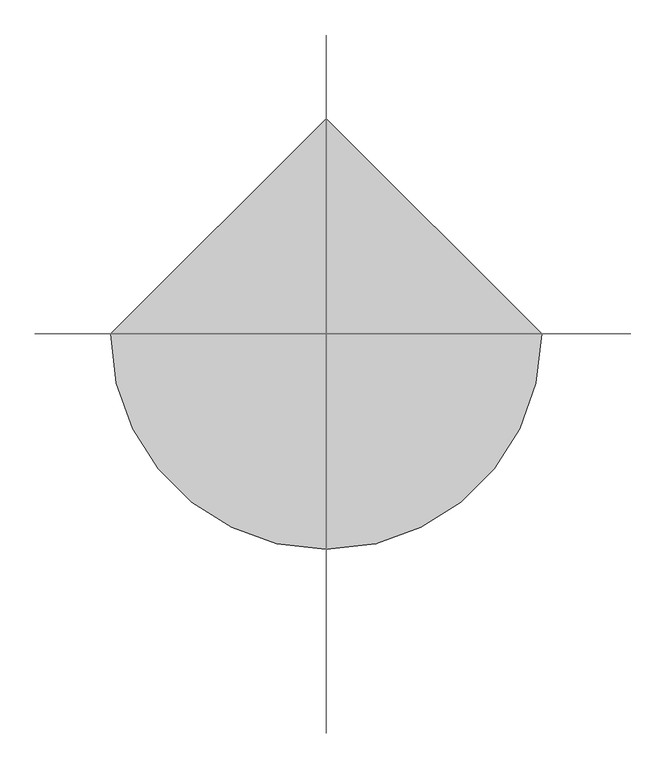
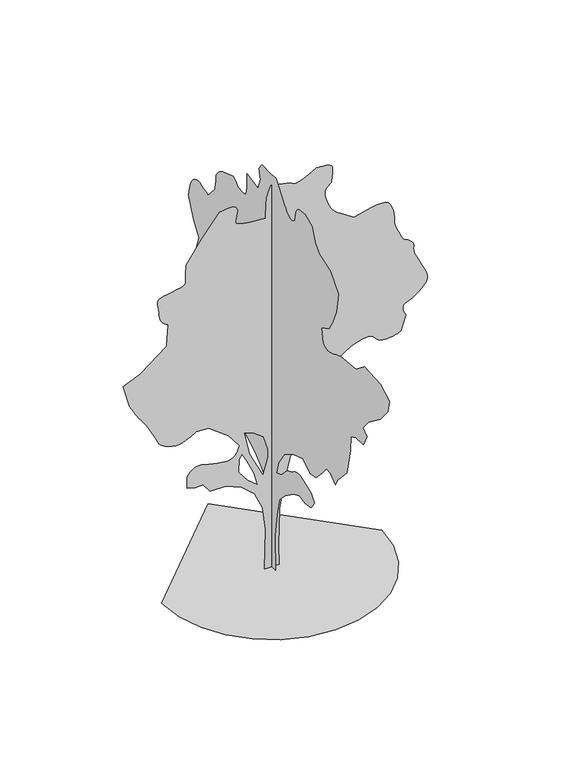
"""IFC4 building model written with IfcOpenShell, lengths in millimetres: proxy geometry, japanese flowering cherry 26172 : japanese flowering cherry 26172."""

import ifcopenshell
import ifcopenshell.guid

model = None  # the IFC model being written
_history = None  # IfcOwnerHistory: only IFC2X3 demands one
_inside = {}  # id of a spatial element -> (the spatial element, [elements in it])
_under = {}  # id of a project, library or spatial element -> (it, [spatial elements below it])
_declared = {}  # id of a project -> (the project, [libraries it declares])
_typed = {}  # id of a type object -> (the type object, [elements of that type])
_made_of = {}  # id of a material, layer set ... -> (it, [elements and type objects made of it])


def new_model(schema):
    """Start an empty IFC model of exactly this schema.

    Asked for "IFC4X3", IfcOpenShell would pick the latest addendum, in which some entities
    have other attributes; the version numbers below select the first issue.
    IFC2X3 requires an IfcOwnerHistory on every rooted entity: one is made here for all.
    """
    global model, _history
    if schema == "IFC4X3":
        model = ifcopenshell.file(schema_version=(4, 3, 0, 0))
    else:
        model = ifcopenshell.file(schema=schema)
    _inside.clear()
    _under.clear()
    _declared.clear()
    _typed.clear()
    _made_of.clear()
    _history = None
    if model.schema == "IFC2X3":
        org = make("IfcOrganization", Name="unknown")
        user = make(
            "IfcPersonAndOrganization",
            ThePerson=make("IfcPerson", FamilyName="unknown"),
            TheOrganization=org,
        )
        app = make(
            "IfcApplication",
            ApplicationDeveloper=org,
            Version="unknown",
            ApplicationFullName="unknown",
            ApplicationIdentifier="unknown",
        )
        _history = make(
            "IfcOwnerHistory",
            OwningUser=user,
            OwningApplication=app,
            ChangeAction="ADDED",
            CreationDate=0,
        )
    return model


def make(cls, **values):
    """One entity of the class cls with the attributes given. An attribute that is None is left unset."""
    return model.create_entity(
        cls, **{name: value for name, value in values.items() if value is not None}
    )


def rooted(cls, **values):
    """An entity with a GlobalId (a new one), such as an element, a storey or a relation."""
    return make(cls, GlobalId=ifcopenshell.guid.new(), OwnerHistory=_history, **values)


def si_unit(unit_type, name, prefix=None):
    """IfcSIUnit, for example si_unit("LENGTHUNIT", "METRE", prefix="MILLI")."""
    return make("IfcSIUnit", UnitType=unit_type, Prefix=prefix, Name=name)


def assignment(units):
    """IfcUnitAssignment: the units of a project."""
    return None if units is None else make("IfcUnitAssignment", Units=units)


def point(xyz):
    """IfcCartesianPoint."""
    return None if xyz is None else make("IfcCartesianPoint", Coordinates=xyz)


def direction(xyz):
    """IfcDirection."""
    return None if xyz is None else make("IfcDirection", DirectionRatios=xyz)


def frame(location, z_axis=None, x_axis=None):
    """IfcAxis2Placement3D, a coordinate frame: its origin and axes. An axis left out is left unset."""
    return make(
        "IfcAxis2Placement3D",
        Location=point(location),
        Axis=direction(z_axis),
        RefDirection=direction(x_axis),
    )


def origin():
    """The frame at (0, 0, 0) with its axes left unset."""
    return frame((0.0, 0.0, 0.0))


def place(relative_to, where):
    """IfcLocalPlacement: puts the frame where relative to a parent placement (None: the world)."""
    return make(
        "IfcLocalPlacement", PlacementRelTo=relative_to, RelativePlacement=where
    )


def context(
    kind, dimensions, precision=None, world=None, true_north=None, identifier=None
):
    """IfcGeometricRepresentationContext, for example the 3D "Model" context."""
    return make(
        "IfcGeometricRepresentationContext",
        ContextIdentifier=identifier,
        ContextType=kind,
        CoordinateSpaceDimension=dimensions,
        Precision=precision,
        WorldCoordinateSystem=world,
        TrueNorth=true_north,
    )


def project(units=None, contexts=None):
    """IfcProject with its units and contexts."""
    return rooted(
        "IfcProject",
        Name="project",
        RepresentationContexts=contexts,
        UnitsInContext=assignment(units),
    )


def spatial(cls, under=None, at=None, **own):
    """A site, building, storey or space (cls), placed at a placement, below another one or the project."""
    s = rooted(cls, ObjectPlacement=at, **own)
    if under is not None:
        _under.setdefault(under.id(), (under, []))[1].append(s)
    return s


def point_list(points):
    """IfcCartesianPointList2D or 3D."""
    cls = (
        "IfcCartesianPointList2D" if len(points[0]) == 2 else "IfcCartesianPointList3D"
    )
    return make(cls, CoordList=points)


def triangles(points, corners, closed=None, point_numbers=None):
    """IfcTriangulatedFaceSet: each triangle names its three corners, points numbered from 1."""
    return make(
        "IfcTriangulatedFaceSet",
        Coordinates=point_list(points),
        Closed=closed,
        CoordIndex=corners,
        PnIndex=point_numbers,
    )


def shape(context_of_items, identifier, shape_type, items):
    """IfcShapeRepresentation: the items that make up one representation, for example the "Body"."""
    return make(
        "IfcShapeRepresentation",
        ContextOfItems=context_of_items,
        RepresentationIdentifier=identifier,
        RepresentationType=shape_type,
        Items=items,
    )


def source(mapping_origin, context_of_items, identifier, shape_type, items):
    """IfcRepresentationMap: a shape defined once, which mapped items show again and again."""
    return make(
        "IfcRepresentationMap",
        MappingOrigin=mapping_origin,
        MappedRepresentation=shape(context_of_items, identifier, shape_type, items),
    )


def transform(
    local_origin,
    x_axis=None,
    y_axis=None,
    z_axis=None,
    scale=None,
    scale2=None,
    scale3=None,
    uniform=True,
):
    """IfcCartesianTransformationOperator3D, or its non-uniform kind. x_axis, y_axis, z_axis: its Axis1, 2, 3."""
    if uniform:
        return make(
            "IfcCartesianTransformationOperator3D",
            Axis1=direction(x_axis),
            Axis2=direction(y_axis),
            LocalOrigin=point(local_origin),
            Scale=scale,
            Axis3=direction(z_axis),
        )
    return make(
        "IfcCartesianTransformationOperator3DnonUniform",
        Axis1=direction(x_axis),
        Axis2=direction(y_axis),
        LocalOrigin=point(local_origin),
        Scale=scale,
        Axis3=direction(z_axis),
        Scale2=scale2,
        Scale3=scale3,
    )


def mapped(mapping_source, mapping_target):
    """IfcMappedItem: shows the shape of a source again, moved by a transform."""
    return make(
        "IfcMappedItem", MappingSource=mapping_source, MappingTarget=mapping_target
    )


def made_of(thing, what):
    """Note that an element or type object is made of a material, layer set ...; save() writes the relation."""
    if what is not None:
        _made_of.setdefault(what.id(), (what, []))[1].append(thing)
    return thing


def element(
    cls,
    number,
    at=None,
    inside=None,
    cuts=None,
    type_object=None,
    material=None,
    context=None,
    identifier="Body",
    shape_type=None,
    held_by="IfcProductDefinitionShape",
    body=None,
    shapes=None,
    **own,
):
    """One element of the class cls, such as IfcWall. Its Tag is "e" and its number.

    at: its placement. inside: the storey or other place that contains it. cuts: it is an
    opening in that element (IfcRelVoidsElement). A single representation is given by context,
    identifier, shape_type and body (its items); several are given by shapes. held_by: the class
    of the entity that holds the representations. save() writes the other relations.
    """
    e = rooted(cls, Tag="e%d" % number, ObjectPlacement=at, **own)
    if body is not None:
        shapes = [shape(context, identifier, shape_type, body)]
    if shapes is not None:
        e.Representation = make(held_by, Representations=shapes)
    if inside is not None:
        _inside.setdefault(inside.id(), (inside, []))[1].append(e)
    if cuts is not None:
        rooted(
            "IfcRelVoidsElement", RelatingBuildingElement=cuts, RelatedOpeningElement=e
        )
    if type_object is not None:
        _typed.setdefault(type_object.id(), (type_object, []))[1].append(e)
    return made_of(e, material)


def aggregate(whole, parts):
    """IfcRelAggregates: a whole, such as a stair, and the parts it consists of."""
    return rooted("IfcRelAggregates", RelatingObject=whole, RelatedObjects=parts)


def save(model, path):
    """Write the relations noted so far, then the file.

    IfcRelAggregates (storeys below a building ...), IfcRelContainedInSpatialStructure (elements
    in a storey), IfcRelDefinesByType, IfcRelAssociatesMaterial and IfcRelDeclares: one each for
    every whole, place, type object, material and project.
    """
    for whole, parts in _under.values():
        aggregate(whole, parts)
    for where, things in _inside.values():
        rooted(
            "IfcRelContainedInSpatialStructure",
            RelatedElements=things,
            RelatingStructure=where,
        )
    for kind, things in _typed.values():
        rooted("IfcRelDefinesByType", RelatedObjects=things, RelatingType=kind)
    for what, things in _made_of.values():
        rooted("IfcRelAssociatesMaterial", RelatedObjects=things, RelatingMaterial=what)
    for by, libraries in _declared.values():
        rooted("IfcRelDeclares", RelatingContext=by, RelatedDefinitions=libraries)
    model.write(path)


def entourage_e499737d(model_context):
    return source(origin(), model_context, "Body", "Tessellation", [
        triangles([(-0.0028028, 75.7657196, 0.0059537), (-0.0028028, -73.2478183, 0.0059537), (-0.0028028, -59.7012251, 399.6312029), (-0.0028028, -100.3410047, 663.7914597), (-0.0028028, -147.7544623, 866.9916292), (-0.0028028, -256.1287339, 982.1375078), (-0.0028028, -418.6863261, 1097.2859299), (-0.0028028, -527.0605977, 1144.6976435), (-0.0028028, -635.434833, 1124.3775902), (-0.0028028, -750.5807842, 1144.6976435), (-0.0028028, -811.5407988, 1232.7519344), (-0.0028028, -750.5807842, 1314.0320023), (-0.0028028, -533.8347845, 1388.5377743), (-0.0028028, -514.9955638, 1387.0189716), (-0.0028028, -496.3341665, 1385.0834793), (-0.0028028, -478.0283798, 1382.3173691), (-0.0028028, -460.2559908, 1378.3091835), (-0.0028028, -443.1947865, 1372.6425236), (-0.0028028, -427.0200471, 1364.9005543), (-0.0028028, -411.9146828, 1354.6719635), (-0.0028028, -396.8067387, 1343.65345), (-0.0028028, -380.6345427, 1333.6991158), (-0.0028028, -363.5733384, 1324.6364422), (-0.0028028, -345.8009494, 1316.2824463), (-0.0028028, -327.4951627, 1308.4643188), (-0.0028028, -308.8337654, 1300.9992222), (-0.0028028, -289.994581, 1293.7118763), (-0.0028028, -188.3942419, 1185.3376774), (-0.0028028, -86.7944115, 1144.6976435), (-0.0028028, -127.4344454, 1286.9377258), (-0.0028028, -242.580869, 1456.2720119), (-0.0028028, -405.140496, 1557.8722057), (-0.0028028, -594.794799, 1618.8321476), (-0.0028028, -730.2607309, 1530.7779293), (-0.0028028, -838.6350025, 1544.3263756), (-0.0028028, -953.7809538, 1666.2439339), (-0.0028028, -1041.8351721, 1774.6181328), (-0.0028028, -1123.1126965, 1767.8439823), (-0.0028028, -1211.1669147, 1686.5663853), (-0.0028028, -1265.3528515, 1781.3922832), (-0.0028028, -1326.3127934, 1849.1240501), (-0.0028028, -1434.6871376, 1964.2723995), (-0.0028028, -1502.4187592, 2269.0726902), (-0.0028028, -1509.193055, 2431.6328259), (-0.0028028, -1604.0214237, 2472.2703163), (-0.0028028, -1753.0332584, 2485.8186172), (-0.0028028, -1813.9932003, 2614.5002975), (-0.0028028, -1739.4874283, 2675.4602394), (-0.0028028, -1841.0874767, 2797.3804138), (-0.0028028, -2071.3792339, 2973.5042564), (-0.0028028, -2220.3935394, 3149.6025192), (-0.0028028, -2247.4851997, 3291.8426743), (-0.0028028, -2078.1535297, 3386.6610146), (-0.0028028, -1766.5790886, 3400.2244308), (-0.0028028, -1610.7931034, 3278.3045471), (-0.0028028, -1312.7669632, 3244.4208595), (-0.0028028, -1272.2845505, 3228.5456657), (-0.0028028, -1232.7519344, 3213.2041603), (-0.0028028, -1195.1115721, 3198.9294502), (-0.0028028, -1160.3186377, 3186.2546425), (-0.0028028, -1129.3153702, 3175.7137161), (-0.0028028, -1103.0517843, 3167.8397781), (-0.0028028, -1082.4726625, 3163.1406464), (-0.0028028, -1064.0500225, 3162.8865921), (-0.0028028, -1044.5580437, 3166.9000099), (-0.0028028, -1025.4242552, 3173.6309944), (-0.0028028, -1008.065867, 3181.5558014), (-0.0028028, -993.907865, 3189.1248161), (-0.0028028, -984.3701477, 3194.789296), (-0.0028028, -980.8726141, 3197.024334), (-0.0028028, -947.0067307, 3359.5844696), (-0.0028028, -1089.2468857, 3434.0828293), (-0.0028028, -1156.9810507, 3542.4645859), (-0.0028028, -1231.4868954, 3718.5628487), (-0.0028028, -1272.127002, 3942.0832169), (-0.0028028, -1116.3410168, 4118.1814796), (-0.0028028, -913.1409199, 4192.7051285), (-0.0028028, -831.8608521, 4267.2034882), (-0.0028028, -770.9007648, 4429.7636238), (-0.0028028, -628.6606825, 4483.9417122), (-0.0028028, -605.4958537, 4483.8402649), (-0.0028028, -582.6891789, 4483.1542603), (-0.0028028, -560.5911455, 4481.2747238), (-0.0028028, -539.5599438, 4477.6426781), (-0.0028028, -519.9511116, 4471.5974075), (-0.0028028, -502.1202959, 4462.6310944), (-0.0028028, -486.4205638, 4450.0836044), (-0.0028028, -473.6824242, 4434.3863068), (-0.0028028, -464.1447433, 4416.5554184), (-0.0028028, -457.2740144, 4396.9467316), (-0.0028028, -452.5343691, 4375.9154572), (-0.0028028, -449.3949532, 4353.8173874), (-0.0028028, -447.3197528, 4331.0083145), (-0.0028028, -445.7805299, 4307.8434494), (-0.0028028, -434.0914178, 4294.9401672), (-0.0028028, -421.9248276, 4283.0531021), (-0.0028028, -408.8133096, 4273.1978897), (-0.0028028, -394.279422, 4266.3398781), (-0.0028028, -377.850701, 4263.5202827), (-0.0028028, -359.0495956, 4265.7303223), (-0.0028028, -337.4062583, 4273.9853416), (-0.0028028, -315.9610193, 4285.9741447), (-0.0028028, -297.7161846, 4298.6995308), (-0.0028028, -282.1358129, 4312.0091835), (-0.0028028, -268.6864885, 4325.8013649), (-0.0028028, -256.8373934, 4339.9237587), (-0.0028028, -246.0563473, 4354.3002068), (-0.0028028, -235.8074452, 4368.8033913), (-0.0028028, -140.9810386, 4497.5054192), (-0.0028028, -80.0209877, 4572.0037788), (-0.0028028, 21.579147, 4565.2219254), (-0.0028028, 184.1389784, 4572.0037788), (-0.0028028, 245.0987749, 4490.7235657), (-0.0028028, 218.0055885, 4375.5852448), (-0.0028028, 265.4200454, 4246.8835075), (-0.0028028, 475.3918765, 4287.5234688), (-0.0028028, 475.3918765, 4138.5014603), (-0.0028028, 476.9514107, 4115.4383331), (-0.0028028, 479.1637756, 4093.1623672), (-0.0028028, 482.6791134, 4072.5630432), (-0.0028028, 488.1502911, 4054.4781006), (-0.0028028, 496.2249435, 4039.6699928), (-0.0028028, 507.5609885, 4029.0273285), (-0.0028028, 522.8060609, 4023.3631393), (-0.0028028, 540.2228757, 4021.2551285), (-0.0028028, 557.6396542, 4020.5691238), (-0.0028028, 575.056469, 4021.0519432), (-0.0028028, 592.4732474, 4022.4995293), (-0.0028028, 609.8900259, 4024.6586998), (-0.0028028, 627.3093842, 4027.2748192), (-0.0028028, 644.726199, 4030.1449928), (-0.0028028, 660.7002239, 4045.9437378), (-0.0028028, 676.7352917, 4060.8791634), (-0.0028028, 692.8896835, 4074.0362091), (-0.0028028, 709.2193554, 4084.5265572), (-0.0028028, 725.7878208, 4091.4607269), (-0.0028028, 742.6534338, 4093.9498192), (-0.0028028, 759.8720776, 4091.1049347), (-0.0028028, 942.7522665, 4030.1449928), (-0.0028028, 968.7009007, 4012.6698967), (-0.0028028, 993.5827394, 3994.8390083), (-0.0028028, 1016.3309875, 3976.2971169), (-0.0028028, 1035.8813931, 3956.6881393), (-0.0028028, 1051.1646172, 3935.6568649), (-0.0028028, 1061.1163353, 3912.8477921), (-0.0028028, 1064.6722956, 3887.9048378), (-0.0028028, 1065.462291, 3862.3526184), (-0.0028028, 1067.6745832, 3837.8921928), (-0.0028028, 1071.0705969, 3814.3209572), (-0.0028028, 1075.4140091, 3791.4610153), (-0.0028028, 1080.4685698, 3769.1088913), (-0.0028028, 1085.9981741, 3747.1381393), (-0.0028028, 1091.7640285, 3725.3447021), (-0.0028028, 1220.4582081, 3583.1045471), (-0.0028028, 1259.5970982, 3600.2497215), (-0.0028028, 1298.4413841, 3615.8705704), (-0.0028028, 1336.691375, 3628.418351), (-0.0028028, 1374.0521759, 3636.343158), (-0.0028028, 1410.2294735, 3638.0956673), (-0.0028028, 1444.9259022, 3632.1521347), (-0.0028028, 1477.8442417, 3616.9629456), (-0.0028028, 1506.4193871, 3593.4931572), (-0.0028028, 1528.9517326, 3564.3086014), (-0.0028028, 1546.4471764, 3530.3996246), (-0.0028028, 1559.9143776, 3492.7059952), (-0.0028028, 1570.361269, 3452.1674812), (-0.0028028, 1578.7941845, 3409.7241417), (-0.0028028, 1586.218586, 3366.3410339), (-0.0028028, 1498.1643677, 3136.0643921), (-0.0028028, 1389.7926395, 2987.0423836), (-0.0028028, 1477.8442417, 2743.2023254), (-0.0028028, 1396.5641739, 2614.5002975), (-0.0028028, 1363.3893093, 2602.8164177), (-0.0028028, 1331.4588455, 2590.6497185), (-0.0028028, 1302.0151485, 2577.543251), (-0.0028028, 1276.3027645, 2563.0144867), (-0.0028028, 1255.5687103, 2546.5806061), (-0.0028028, 1241.0552067, 2527.7820442), (-0.0028028, 1234.0040382, 2506.1385979), (-0.0028028, 1231.6953129, 2483.1135498), (-0.0028028, 1230.4506214, 2460.4416779), (-0.0028028, 1230.0949745, 2438.0692062), (-0.0028028, 1230.4506214, 2415.9330574), (-0.0028028, 1231.339666, 2393.9721886), (-0.0028028, 1232.5842121, 2372.13326), (-0.0028028, 1234.0040382, 2350.3502872), (-0.0028028, 1206.9124506, 2241.9785591), (-0.0028028, 1017.2581112, 2262.2985397), (-0.0028028, 1001.4999161, 2230.5052769), (-0.0028028, 986.9863398, 2199.5401611), (-0.0028028, 974.9594576, 2170.2361359), (-0.0028028, 966.6663591, 2143.4188774), (-0.0028028, 963.3491198, 2119.9211838), (-0.0028028, 966.2523582, 2100.5664059), (-0.0028028, 976.6180773, 2086.1925739), (-0.0028028, 993.4227201, 2074.2646683), (-0.0028028, 1014.0196461, 2062.1005852), (-0.0028028, 1037.2225176, 2050.292149), (-0.0028028, 1061.8478313, 2039.431184), (-0.0028028, 1086.7093952, 2030.1093693), (-0.0028028, 1110.6234879, 2022.9211452), (-0.0028028, 1132.4039898, 2018.4583363), (-0.0028028, 1152.1322187, 2014.567004), (-0.0028028, 1170.7936523, 2008.9003441), (-0.0028028, 1188.5660414, 2001.7526699), (-0.0028028, 1205.6272093, 1993.4190216), (-0.0028028, 1222.157523, 1984.1961834), (-0.0028028, 1238.3297916, 1974.3816662), (-0.0028028, 1254.3241642, 1964.2723995), (-0.0028028, 1410.1126202, 2045.5524673), (-0.0028028, 1454.8979679, 2056.9850544), (-0.0028028, 1498.4412403, 2067.3533169), (-0.0028028, 1539.4952751, 2075.5879887), (-0.0028028, 1576.817997, 2080.6222744), (-0.0028028, 1609.1650051, 2081.3919949), (-0.0028028, 1635.2914627, 2076.8326801), (-0.0028028, 1653.9502075, 2065.8725933), (-0.0028028, 1666.2946575, 2049.9747265), (-0.0028028, 1674.7249569, 2031.5900928), (-0.0028028, 1679.8989143, 2011.1329113), (-0.0028028, 1682.4669262, 1989.0146393), (-0.0028028, 1683.0789528, 1965.6542919), (-0.0028028, 1682.3881519, 1941.4631813), (-0.0028028, 1681.0444839, 1916.8582878), (-0.0028028, 1657.7627655, 1892.3904499), (-0.0028028, 1634.1255455, 1869.1697742), (-0.0028028, 1609.7770317, 1848.4331039), (-0.0028028, 1584.3618679, 1831.4303627), (-0.0028028, 1557.5241165, 1819.4059513), (-0.0028028, 1528.9110374, 1813.5996197), (-0.0028028, 1498.1643677, 1815.2582394), (-0.0028028, 1465.6015297, 1822.4057682), (-0.0028028, 1432.5637207, 1830.9782101), (-0.0028028, 1400.2370602, 1839.0732101), (-0.0028028, 1369.8078129, 1844.8009129), (-0.0028028, 1342.4571568, 1846.2614342), (-0.0028028, 1319.3735367, 1841.5624477), (-0.0028028, 1301.7382759, 1828.8040695), (-0.0028028, 1288.4084209, 1812.3752758), (-0.0028028, 1277.2120113, 1797.7219551), (-0.0028028, 1267.7912201, 1784.5521194), (-0.0028028, 1259.7953419, 1772.5657871), (-0.0028028, 1252.8636429, 1761.4660286), (-0.0028028, 1246.6430923, 1750.9605652), (-0.0028028, 1240.778334, 1740.752322), (-0.0028028, 1263.8618088, 1737.6916077), (-0.0028028, 1286.1172817, 1733.6834221), (-0.0028028, 1306.714135, 1727.7779686), (-0.0028028, 1324.821896, 1719.0302467), (-0.0028028, 1339.6122723, 1706.4901691), (-0.0028028, 1350.2574074, 1689.2105553), (-0.0028028, 1355.9242126, 1666.2439339), (-0.0028028, 1358.2355541, 1639.3300243), (-0.0028028, 1359.4802456, 1610.9912018), (-0.0028028, 1359.8357471, 1581.4687305), (-0.0028028, 1359.4802456, 1550.9989334), (-0.0028028, 1358.591201, 1519.8178425), (-0.0028028, 1357.3466549, 1488.1643967), (-0.0028028, 1355.9242126, 1456.2720119), (-0.0028028, 1321.1312782, 1430.3436527), (-0.0028028, 1286.5720505, 1405.5990875), (-0.0028028, 1252.4876484, 1383.2266159), (-0.0028028, 1219.1146128, 1364.4078518), (-0.0028028, 1186.6915192, 1350.328624), (-0.0028028, 1155.4494581, 1342.1725811), (-0.0028028, 1125.6323828, 1341.1261333), (-0.0028028, 1095.812764, 1344.8167511), (-0.0028028, 1064.5732464, 1349.9322819), (-0.0028028, 1032.1476093, 1356.2316067), (-0.0028028, 998.774501, 1363.478112), (-0.0028028, 964.6902443, 1371.4385273), (-0.0028028, 930.1334873, 1379.8688267), (-0.0028028, 895.3380095, 1388.5377743), (-0.0028028, 692.1378399, 1341.1261333), (-0.0028028, 455.0718596, 1219.2061043), (-0.0028028, 319.6059277, 1144.6976435), (-0.0028028, 163.8189614, 1016.005862), (-0.0028028, 68.9922959, 819.5799156), (-0.0028028, 41.8991095, 541.8713216), (-0.0028028, 68.9922959, 264.1652892), (80.2102203, 0.0002552, 0.0), (-82.349661, 0.0002552, 0.0), (-68.8030678, 0.0002233, 460.5862032), (-102.6694236, 0.000202, 724.7463873), (-190.7229152, 0.0001914, 914.3981833), (-332.9637969, 0.0001914, 1043.0925081), (-509.0697627, 0.0001807, 1117.5983528), (-678.4015417, 0.0001807, 1117.5983528), (-759.684153, 0.0001807, 1219.1984013), (-847.7358278, 0.0001807, 1219.1984013), (-935.7901188, 0.0001807, 1239.5183819), (-935.7901188, 0.0001701, 1368.2127068), (-918.2539072, 0.0001701, 1391.2175526), (-900.0065472, 0.0001701, 1412.9192802), (-880.3392883, 0.0001595, 1432.0150623), (-858.5384388, 0.0001595, 1447.2017807), (-833.8928501, 0.0001595, 1457.1737011), (-805.6936993, 0.0001595, 1460.6307575), (-773.2299831, 0.0001595, 1456.266925), (-734.6829174, 0.0001595, 1446.5108345), (-690.4487715, 0.0001595, 1435.4516258), (-643.1335636, 0.0001701, 1424.2757092), (-595.3460009, 0.0001701, 1414.1639717), (-549.689449, 0.0001701, 1406.3051491), (-508.7725788, 0.0001701, 1401.8804192), (-475.2013721, 0.0001701, 1402.0785175), (-448.544024, 0.0001701, 1408.1415195), (-426.1513865, 0.0001701, 1419.8916744), (-407.3122021, 0.0001595, 1436.3813656), (-391.3152497, 0.0001595, 1456.660651), (-377.4544679, 0.0001595, 1479.7848209), (-365.0135485, 0.0001595, 1504.8039333), (-353.2838139, 0.0001595, 1530.7728424), (-475.2013721, 0.0001488, 1693.3329781), (-698.7215223, 0.0001382, 1855.8931137), (-834.1899977, 0.0001382, 1862.6647934), (-856.0492739, 0.0001382, 1849.6320133), (-878.4419477, 0.0001382, 1836.7771294), (-901.9038877, 0.0001382, 1824.277747), (-926.9610065, 0.0001382, 1812.3092915), (-954.1543322, 0.0001382, 1801.0544552), (-984.01203, 0.0001382, 1790.6861927), (-1017.0701866, 0.0001488, 1781.3847256), (-1055.1015862, 0.0001488, 1778.1664627), (-1097.4002398, 0.0001488, 1784.6638859), (-1140.7656887, 0.0001382, 1798.9792912), (-1182.0000904, 0.0001382, 1819.2206429), (-1217.9005154, 0.0001382, 1843.490237), (-1245.2690483, 0.0001382, 1869.8935673), (-1260.907774, 0.0001382, 1896.5332203), (-1274.5551968, 0.0001382, 1929.7461639), (-1296.2570698, 0.0001276, 1973.9803825), (-1323.2903034, 0.0001276, 2024.4959038), (-1352.9320988, 0.0001276, 2076.5482498), (-1382.45457, 0.0001276, 2125.4025352), (-1409.1321568, 0.0001169, 2166.3195145), (-1430.2420601, 0.0001169, 2194.5592152), (-1448.055217, 0.0001169, 2217.0508656), (-1466.5769062, 0.0001169, 2243.4541958), (-1485.6928905, 0.0001169, 2273.113868), (-1505.2813751, 0.0001169, 2305.3794857), (-1525.2255066, 0.0001063, 2339.6035595), (-1545.4082863, 0.0001063, 2375.12799), (-1565.7080647, 0.0001063, 2411.3051422), (-1640.2164528, 9.57e-05, 2668.7039658), (-1443.7878902, 8.51e-05, 2749.9838882), (-1159.310269, 7.44e-05, 2973.5042564), (-1145.7618954, 5.32e-05, 3217.3190254), (-1165.9447477, 5.32e-05, 3231.9748169), (-1185.2970549, 5.32e-05, 3247.3163223), (-1202.9906696, 5.32e-05, 3264.0804153), (-1218.1951195, 5.32e-05, 3282.9780991), (-1230.0823299, 5.32e-05, 3304.7203766), (-1237.8242992, 5.32e-05, 3330.0188324), (-1240.5902641, 5.32e-05, 3359.5591805), (-1243.0389519, 4.25e-05, 3392.8330215), (-1248.5659401, 4.25e-05, 3427.5294502), (-1254.4511913, 4.25e-05, 3461.7686394), (-1257.9665291, 4.25e-05, 3493.6204742), (-1256.3865383, 4.25e-05, 3521.204837), (-1246.9860947, 4.25e-05, 3542.6169022), (-1227.0419632, 4.25e-05, 3556.002713), (-1192.1092844, 4.25e-05, 3564.4103394), (-1144.1438982, 3.19e-05, 3572.715937), (-1090.0164608, 3.19e-05, 3581.5808029), (-1036.6002445, 3.19e-05, 3591.7915169), (-990.7659056, 3.19e-05, 3603.9835052), (-959.3867163, 3.19e-05, 3618.9186401), (-949.3359489, 3.19e-05, 3637.2829262), (-951.449192, 3.19e-05, 3659.3809959), (-952.1400656, 3.19e-05, 3684.6794518), (-951.644747, 3.19e-05, 3712.6448959), (-950.2045732, 3.19e-05, 3742.718351), (-948.0532511, 2.13e-05, 3774.4175789), (-945.4268852, 2.13e-05, 3807.1836021), (-942.5617258, 2.13e-05, 3840.4830231), (-773.2299831, 1.06e-05, 4084.3233719), (-576.803964, -1.06e-05, 4328.16343), (-534.9980856, -1.06e-05, 4335.1231796), (-494.9117606, -1.06e-05, 4340.3809982), (-458.2595647, -1.06e-05, 4342.2096657), (-426.7635221, -1.06e-05, 4338.8569633), (-402.1382083, -1.06e-05, 4328.6459587), (-386.1031769, -1.06e-05, 4309.850013), (-380.3754742, 0.0, 4280.7416153), (-383.1999384, 0.0, 4247.9503029), (-389.6972889, 0.0, 4219.0450905), (-396.9057878, 0.0, 4193.848082), (-401.8613357, 0.0, 4172.0549355), (-401.6048106, 0.0, 4153.462175), (-393.1720041, 0.0, 4137.8410355), (-373.6038308, 0.0, 4124.9633331), (-343.9238837, 0.0, 4114.5238541), (-307.8431645, 0.0, 4106.2435455), (-266.4335192, 1.06e-05, 4099.7157463), (-220.7586908, 1.06e-05, 4094.6355331), (-171.883967, 1.06e-05, 4090.5971169), (-120.8766607, 1.06e-05, 4087.2697037), (-68.8030678, 1.06e-05, 4084.3233719), (-62.0293897, 0.0, 4267.2034882), (-60.4495079, -1.06e-05, 4293.1367889), (-56.0260951, -1.06e-05, 4318.689299), (-49.2331141, -1.06e-05, 4343.962175), (-40.544273, -1.06e-05, 4369.0065765), (-30.4335416, -1.06e-05, 4393.8733727), (-19.3751868, -1.06e-05, 4418.612851), (-7.8427643, -1.06e-05, 4443.3017509), (38.3857792, -1.06e-05, 4434.5642029), (83.3110485, -1.06e-05, 4425.7249168), (125.6295138, -1.06e-05, 4416.6571564), (164.0381523, -1.06e-05, 4407.2083145), (197.2334371, -1.06e-05, 4397.3022331), (223.9120957, -1.06e-05, 4386.7865959), (242.7705922, -1.06e-05, 4375.5599556), (267.3174405, -1.06e-05, 4372.2834114), (307.2640574, -1.06e-05, 4382.5194145), (355.6256767, -1.06e-05, 4401.5188362), (405.4097383, -1.06e-05, 4424.5566742), (449.6235366, -1.06e-05, 4446.8576385), (481.2770551, -2.13e-05, 4463.7234695), (493.3827115, -2.13e-05, 4470.4035851), (503.1388384, -2.13e-05, 4470.6067703), (528.2975498, -2.13e-05, 4470.3274269), (562.6967946, -2.13e-05, 4468.2699944), (600.177065, -2.13e-05, 4463.1392029), (634.5763098, -1.06e-05, 4453.6142029), (659.7350212, -1.06e-05, 4438.3994339), (669.4911844, -1.06e-05, 4416.1999168), (669.0949877, -1.06e-05, 4390.4698013), (667.9900406, -1.06e-05, 4365.4506889), (666.2907984, -1.06e-05, 4341.0411324), (664.1190559, -1.06e-05, 4317.089106), (661.5918119, -1.06e-05, 4293.4922905), (658.8257017, 0.0, 4270.1245308), (655.9428108, 0.0, 4246.8835075), (638.6835445, 0.0, 4233.6753021), (622.3741476, 0.0, 4219.7308044), (607.9571134, 0.0, 4204.2114029), (596.3848546, 0.0, 4186.4060944), (588.6048426, 0.0, 4165.5271362), (585.5644395, 0.0, 4140.7876579), (588.2111166, 0.0, 4111.3996262), (595.5949319, 1.06e-05, 4078.8367882), (605.8235227, 1.06e-05, 4045.6643944), (618.4244614, 1.06e-05, 4012.9492401), (632.9176901, 1.06e-05, 3981.7834099), (648.8333611, 1.06e-05, 3953.233699), (665.698974, 1.06e-05, 3928.3416138), (683.0370146, 2.13e-05, 3908.1995293), (703.4154945, 2.13e-05, 3889.8099541), (729.1278786, 2.13e-05, 3869.6170006), (759.2802532, 2.13e-05, 3847.9505905), (792.9912043, 2.13e-05, 3825.1159378), (829.3639841, 2.13e-05, 3801.3670967), (867.5148531, 2.13e-05, 3777.0592781), (906.5572374, 2.13e-05, 3752.4212471), (974.48703, 2.13e-05, 3771.0140076), (1040.6997763, 2.13e-05, 3787.8795479), (1103.475959, 2.13e-05, 3801.2909386), (1161.1010027, 2.13e-05, 3809.5712471), (1211.8502306, 2.13e-05, 3810.9682549), (1254.0116833, 2.13e-05, 3803.7800308), (1285.8633728, 2.13e-05, 3786.2793549), (1308.8096466, 2.13e-05, 3757.831382), (1325.9495888, 3.19e-05, 3721.2045479), (1338.1136719, 3.19e-05, 3679.8280037), (1346.1325138, 3.19e-05, 3637.155899), (1350.8315002, 3.19e-05, 3596.6173851), (1353.0438652, 4.25e-05, 3561.641613), (1353.5976105, 4.25e-05, 3535.6827324), (1358.8503422, 4.25e-05, 3507.9969223), (1372.3961723, 4.25e-05, 3469.2870758), (1390.9178616, 4.25e-05, 3425.1418053), (1411.1006413, 5.32e-05, 3381.0982727), (1429.6249466, 5.32e-05, 3342.7442184), (1443.1707767, 5.32e-05, 3315.6423843), (1448.4235085, 5.32e-05, 3305.3808014), (1455.5126106, 5.32e-05, 3302.5614967), (1473.6202263, 5.32e-05, 3294.4079247), (1498.0094353, 5.32e-05, 3281.4031952), (1523.9376492, 5.32e-05, 3264.0042572), (1546.6656223, 5.32e-05, 3242.6936394), (1561.456144, 5.32e-05, 3217.9538704), (1563.5693871, 6.38e-05, 3190.2424805), (1560.9227463, 6.38e-05, 3161.8962456), (1563.9655838, 6.38e-05, 3134.3880409), (1571.7456322, 6.38e-05, 3106.8795456), (1583.3178909, 6.38e-05, 3078.5585999), (1597.7324181, 6.38e-05, 3048.5613029), (1614.0443584, 7.44e-05, 3016.0746231), (1631.3036247, 7.44e-05, 2980.2605301), (1651.0114334, 7.44e-05, 2941.4239471), (1672.8529781, 7.44e-05, 2900.911013), (1693.1526112, 7.44e-05, 2859.5850471), (1708.2377369, 8.51e-05, 2818.2593719), (1714.4404106, 8.51e-05, 2777.7461472), (1708.0801884, 8.51e-05, 2738.9095642), (1685.4894161, 8.51e-05, 2702.5620735), (1655.0603142, 9.57e-05, 2670.8884254), (1626.9983643, 9.57e-05, 2644.9042557), (1600.3587112, 9.57e-05, 2623.6442162), (1574.1941746, 9.57e-05, 2606.1944092), (1547.5546669, 9.57e-05, 2591.5894867), (1519.4951878, 9.57e-05, 2578.8641006), (1489.0634697, 9.57e-05, 2567.103772), (1463.2545799, 9.57e-05, 2553.5147758), (1448.4615875, 9.57e-05, 2536.3646599), (1442.8532089, 9.57e-05, 2516.2632706), (1444.5930737, 0.0001063, 2493.7893517), (1451.8397243, 0.0001063, 2469.5399597), (1462.7592613, 0.0001063, 2444.1069191), (1475.5176395, 0.0001063, 2418.079438), (1421.329232, 0.0001169, 2248.7450066), (1402.2741451, 0.0001169, 2240.1167542), (1382.0913654, 0.0001169, 2231.9607113), (1359.6579964, 0.0001169, 2224.752285), (1333.8491066, 0.0001169, 2218.9661556), (1303.5367126, 0.0001169, 2215.0772942), (1267.5955925, 0.0001169, 2213.5558754), (1224.9032856, 0.0001169, 2214.8791958), (1186.5543182, 0.0001169, 2223.6651421), (1160.2907324, 0.0001169, 2241.2216286), (1139.9504042, 0.0001169, 2263.0426804), (1119.3738258, 0.0001169, 2284.6250839), (1092.3990189, 0.0001169, 2301.470422), (1052.8638594, 0.0001169, 2309.0727196), (994.6089123, 0.0001169, 2302.9309433), (927.2531399, 0.0001169, 2283.7970821), (865.4625074, 0.0001169, 2256.8426228), (810.6645441, 0.0001169, 2224.1985397), (764.2764599, 0.0001169, 2188.0035107), (727.7258566, 0.0001169, 2150.3835686), (702.4274008, 0.0001276, 2113.4772457), (689.8112377, 0.0001276, 2079.4133366), (689.5343651, 0.0001276, 2049.0602474), (699.2092106, 0.0001276, 2021.5520428), (717.179698, 0.0001276, 1996.4136063), (741.7847368, 0.0001276, 1973.172583), (771.3655621, 0.0001382, 1951.3515312), (804.2662428, 0.0001382, 1930.4778053), (838.8229998, 0.0001382, 1910.0790504), (858.9855045, 0.0001382, 1896.9268009), (878.2006107, 0.0001382, 1883.2412991), (895.5183764, 0.0001382, 1868.4914726), (909.9938009, 0.0001382, 1852.1415985), (920.6770878, 0.0001382, 1833.6579884), (926.620693, 0.0001382, 1812.5073898), (926.8772181, 0.0001382, 1788.158876), (924.1721506, 0.0001488, 1758.4790016), (921.8225847, 0.0001488, 1722.4008259), (919.7677683, 0.0001488, 1680.9911442), (917.9516727, 0.0001488, 1635.3142811), (916.3107845, 0.0001595, 1586.4395027), (914.7919092, 0.0001595, 1535.4337498), (913.3288445, 0.0001595, 1483.3585854), (878.4571358, 0.0001595, 1457.529348), (843.3467062, 0.0001595, 1433.4780544), (807.7613056, 0.0001701, 1412.980323), (771.4646839, 0.0001701, 1397.8139523), (734.2231344, 0.0001701, 1389.7570312), (695.792922, 0.0001701, 1390.585033), (655.9428108, 0.0001701, 1402.0785175), (615.8971447, 0.0001701, 1417.3236626), (576.9157305, 0.0001701, 1428.6597439), (538.820781, 0.0001595, 1436.7368671), (501.4395962, 0.0001595, 1442.205574), (464.5917727, 0.0001595, 1445.7209118), (428.0995597, 0.0001595, 1447.9332767), (391.7826267, 0.0001595, 1449.4927746), (276.6366936, 0.0001701, 1374.9868572), (202.1305764, 0.0001807, 1205.6525711), (127.6236689, 0.0001914, 921.1724064), (86.9838894, 0.0002126, 643.4663195), (73.4370464, 0.0002339, 237.0665254), (-95.8962542, 8.51e-05, 1097.2783722), (-41.7096271, 7.44e-05, 1286.9326389), (-41.7096271, 6.38e-05, 1381.7585369), (-89.122576, 5.32e-05, 1544.3186726), (-211.0424234, 5.32e-05, 1632.3728909), (-305.8695931, 5.32e-05, 1666.238847), (-244.9095423, 6.38e-05, 1395.3069832), (-156.8557963, 6.38e-05, 1009.2266247), (-197.4958302, 6.38e-05, 1158.2383867), (-272.003746, 5.32e-05, 1320.7984497), (-326.1896101, 4.25e-05, 1422.3986435), (-360.0554572, 4.25e-05, 1374.9868572), (-366.829644, 5.32e-05, 1225.9725517), (-265.2295592, 6.38e-05, 1097.2783722), (-1212.9170259, 0.0, 0.0045929), (-1180.85205, -277.9194097, 0.0045929), (-1089.5287725, -533.1464181, 0.0045929), (-946.2625174, -758.3633034, 0.0045929), (-758.3633034, -946.2625174, 0.0045929), (-533.1464181, -1089.5287725, 0.0045929), (-277.9194097, -1180.85205, 0.0045929), (5.3e-05, -1212.9170259, 0.0045929), (277.9194097, -1180.85205, 0.0045929), (533.1464181, -1089.5287725, 0.0045929), (758.3633034, -946.2625174, 0.0045929), (946.2625174, -758.3633034, 0.0045929), (1089.5287725, -533.1464181, 0.0045929), (1180.85205, -277.9194097, 0.0045929), (1212.9170259, 0.0001063, 0.0045929), (-0.0001591, 1212.9170259, 0.0045929)], [[38, 39, 40], [115, 116, 117], [1, 2, 3], [280, 1, 3], [279, 280, 3], [279, 3, 4], [278, 279, 4], [278, 4, 5], [186, 187, 188], [277, 278, 5], [46, 47, 48], [45, 46, 48], [277, 5, 6], [185, 186, 188], [10, 11, 12], [9, 10, 12], [9, 12, 13], [8, 9, 13], [8, 13, 14], [8, 14, 15], [8, 15, 16], [8, 16, 17], [8, 17, 18], [8, 18, 19], [8, 19, 20], [8, 20, 21], [7, 8, 21], [7, 21, 22], [7, 22, 23], [7, 23, 24], [7, 24, 25], [7, 25, 26], [6, 7, 26], [6, 26, 27], [6, 27, 28], [277, 6, 28], [277, 28, 29], [51, 52, 53], [50, 51, 53], [50, 53, 54], [50, 54, 55], [49, 50, 55], [49, 55, 56], [48, 49, 56], [48, 56, 57], [45, 48, 57], [44, 45, 57], [44, 57, 58], [44, 58, 59], [44, 59, 60], [44, 60, 61], [44, 61, 62], [44, 62, 63], [276, 277, 29], [276, 29, 30], [184, 185, 188], [183, 184, 188], [44, 63, 64], [115, 117, 118], [111, 112, 113], [111, 113, 114], [182, 183, 188], [109, 110, 111], [109, 111, 114], [108, 109, 114], [108, 114, 115], [107, 108, 115], [106, 107, 115], [105, 106, 115], [104, 105, 115], [115, 118, 119], [170, 171, 172], [170, 172, 173], [170, 173, 174], [170, 174, 175], [74, 75, 76], [74, 76, 77], [73, 74, 77], [72, 73, 77], [71, 72, 77], [258, 259, 260], [181, 182, 188], [78, 79, 80], [170, 175, 176], [103, 104, 115], [78, 80, 81], [44, 64, 65], [275, 276, 30], [275, 30, 31], [274, 275, 31], [78, 81, 82], [78, 82, 83], [78, 83, 84], [78, 84, 85], [78, 85, 86], [78, 86, 87], [78, 87, 88], [78, 88, 89], [78, 89, 90], [78, 90, 91], [78, 91, 92], [78, 92, 93], [78, 93, 94], [78, 94, 95], [78, 95, 96], [71, 77, 78], [71, 78, 96], [71, 96, 97], [71, 97, 98], [71, 98, 99], [71, 99, 100], [115, 119, 120], [180, 181, 188], [38, 40, 41], [223, 224, 225], [33, 34, 35], [33, 35, 36], [33, 36, 37], [102, 103, 115], [179, 180, 188], [44, 65, 66], [170, 176, 177], [71, 100, 101], [43, 44, 66], [42, 43, 66], [41, 42, 66], [38, 41, 66], [37, 38, 66], [33, 37, 66], [33, 66, 67], [33, 67, 68], [33, 68, 69], [33, 69, 70], [32, 33, 70], [31, 32, 70], [274, 31, 70], [273, 274, 70], [273, 70, 71], [273, 71, 101], [273, 101, 102], [273, 102, 115], [273, 115, 120], [273, 120, 121], [273, 121, 122], [273, 122, 123], [273, 123, 124], [273, 124, 125], [273, 125, 126], [273, 126, 127], [273, 127, 128], [273, 128, 129], [273, 129, 130], [273, 130, 131], [272, 273, 131], [271, 272, 131], [270, 271, 131], [269, 270, 131], [268, 269, 131], [268, 131, 132], [268, 132, 133], [268, 133, 134], [167, 168, 169], [257, 258, 260], [257, 260, 261], [256, 257, 261], [256, 261, 262], [255, 256, 262], [255, 262, 263], [254, 255, 263], [254, 263, 264], [254, 264, 265], [254, 265, 266], [254, 266, 267], [254, 267, 268], [253, 254, 268], [252, 253, 268], [251, 252, 268], [250, 251, 268], [249, 250, 268], [248, 249, 268], [247, 248, 268], [246, 247, 268], [245, 246, 268], [166, 167, 169], [165, 166, 169], [164, 165, 169], [163, 164, 169], [162, 163, 169], [161, 162, 169], [160, 161, 169], [159, 160, 169], [158, 159, 169], [157, 158, 169], [156, 157, 169], [155, 156, 169], [154, 155, 169], [154, 169, 170], [154, 170, 177], [153, 154, 177], [153, 177, 178], [153, 178, 179], [153, 179, 188], [222, 223, 225], [222, 225, 226], [221, 222, 226], [220, 221, 226], [219, 220, 226], [218, 219, 226], [217, 218, 226], [216, 217, 226], [215, 216, 226], [214, 215, 226], [213, 214, 226], [212, 213, 226], [212, 226, 227], [212, 227, 228], [212, 228, 229], [212, 229, 230], [212, 230, 231], [211, 212, 231], [211, 231, 232], [211, 232, 233], [210, 211, 233], [209, 210, 233], [209, 233, 234], [209, 234, 235], [209, 235, 236], [209, 236, 237], [209, 237, 238], [209, 238, 239], [209, 239, 240], [208, 209, 240], [208, 240, 241], [207, 208, 241], [206, 207, 241], [206, 241, 242], [205, 206, 242], [204, 205, 242], [204, 242, 243], [203, 204, 243], [202, 203, 243], [202, 243, 244], [201, 202, 244], [201, 244, 245], [201, 245, 268], [200, 201, 268], [199, 200, 268], [198, 199, 268], [197, 198, 268], [196, 197, 268], [195, 196, 268], [194, 195, 268], [153, 188, 189], [153, 189, 190], [152, 153, 190], [152, 190, 191], [151, 152, 191], [136, 137, 138], [135, 136, 138], [135, 138, 139], [134, 135, 139], [134, 139, 140], [134, 140, 141], [134, 141, 142], [134, 142, 143], [134, 143, 144], [134, 144, 145], [134, 145, 146], [134, 146, 147], [134, 147, 148], [134, 148, 149], [134, 149, 150], [134, 150, 151], [134, 151, 191], [134, 191, 192], [134, 192, 193], [268, 134, 193], [194, 268, 193], [583, 580, 581], [574, 281, 575], [580, 583, 584], [573, 574, 575], [583, 581, 575], [580, 584, 585], [572, 573, 575], [582, 583, 575], [582, 575, 281], [571, 572, 575], [571, 575, 576], [281, 282, 283], [570, 571, 576], [570, 576, 577], [344, 345, 346], [290, 291, 292], [406, 407, 408], [570, 577, 578], [290, 292, 293], [289, 290, 293], [289, 293, 294], [289, 294, 295], [289, 295, 296], [289, 296, 297], [289, 297, 298], [289, 298, 299], [289, 299, 300], [289, 300, 301], [289, 301, 302], [289, 302, 303], [288, 289, 303], [287, 288, 303], [287, 303, 304], [287, 304, 305], [287, 305, 306], [286, 287, 306], [286, 306, 307], [286, 307, 308], [286, 308, 309], [569, 570, 578], [554, 555, 556], [405, 406, 408], [343, 344, 346], [512, 513, 514], [511, 512, 514], [511, 514, 515], [511, 515, 516], [511, 516, 517], [510, 511, 517], [510, 517, 518], [510, 518, 519], [510, 519, 520], [510, 520, 521], [510, 521, 522], [510, 522, 523], [510, 523, 524], [509, 510, 524], [509, 524, 525], [508, 509, 525], [434, 435, 436], [342, 343, 346], [507, 508, 525], [507, 525, 526], [405, 408, 409], [404, 405, 409], [403, 404, 409], [403, 409, 410], [402, 403, 410], [401, 402, 410], [400, 401, 410], [400, 410, 411], [399, 400, 411], [399, 411, 412], [399, 412, 413], [399, 413, 414], [399, 414, 415], [377, 378, 379], [341, 342, 346], [341, 346, 347], [340, 341, 347], [339, 340, 347], [338, 339, 347], [337, 338, 347], [336, 337, 347], [335, 336, 347], [334, 335, 347], [333, 334, 347], [377, 379, 380], [377, 380, 381], [377, 381, 382], [377, 382, 383], [377, 383, 384], [377, 384, 385], [377, 385, 386], [377, 386, 387], [377, 387, 388], [377, 388, 389], [377, 389, 390], [377, 390, 391], [376, 377, 391], [376, 391, 392], [375, 376, 392], [374, 375, 392], [373, 374, 392], [372, 373, 392], [372, 392, 393], [371, 372, 393], [370, 371, 393], [369, 370, 393], [369, 393, 394], [369, 394, 395], [369, 395, 396], [332, 333, 347], [369, 396, 397], [426, 427, 428], [426, 428, 429], [425, 426, 429], [425, 429, 430], [424, 425, 430], [424, 430, 431], [423, 424, 431], [423, 431, 432], [422, 423, 432], [422, 432, 433], [421, 422, 433], [420, 421, 433], [419, 420, 433], [418, 419, 433], [418, 433, 434], [418, 434, 436], [418, 436, 437], [418, 437, 438], [418, 438, 439], [417, 418, 439], [417, 439, 440], [416, 417, 440], [416, 440, 441], [415, 416, 441], [399, 415, 441], [399, 441, 442], [399, 442, 443], [399, 443, 444], [399, 444, 445], [399, 445, 446], [399, 446, 447], [399, 447, 448], [399, 448, 449], [369, 397, 398], [331, 332, 347], [368, 369, 398], [360, 361, 362], [359, 360, 362], [359, 362, 363], [358, 359, 363], [358, 363, 364], [357, 358, 364], [357, 364, 365], [356, 357, 365], [355, 356, 365], [355, 365, 366], [354, 355, 366], [353, 354, 366], [352, 353, 366], [351, 352, 366], [350, 351, 366], [349, 350, 366], [348, 349, 366], [348, 366, 367], [348, 367, 368], [348, 368, 398], [347, 348, 398], [347, 398, 399], [347, 399, 449], [347, 449, 450], [347, 450, 451], [347, 451, 452], [331, 347, 452], [331, 452, 453], [331, 453, 454], [331, 454, 455], [331, 455, 456], [330, 331, 456], [329, 330, 456], [328, 329, 456], [327, 328, 456], [326, 327, 456], [325, 326, 456], [324, 325, 456], [323, 324, 456], [322, 323, 456], [321, 322, 456], [320, 321, 456], [319, 320, 456], [318, 319, 456], [317, 318, 456], [316, 317, 456], [315, 316, 456], [314, 315, 456], [314, 456, 457], [314, 457, 458], [314, 458, 459], [314, 459, 460], [314, 460, 461], [314, 461, 462], [314, 462, 463], [314, 463, 464], [314, 464, 465], [314, 465, 466], [314, 466, 467], [314, 467, 468], [314, 468, 469], [314, 469, 470], [314, 470, 471], [314, 471, 472], [314, 472, 473], [314, 473, 474], [314, 474, 475], [314, 475, 476], [314, 476, 477], [314, 477, 478], [314, 478, 479], [314, 479, 480], [314, 480, 481], [314, 481, 482], [314, 482, 483], [314, 483, 484], [314, 484, 485], [314, 485, 486], [314, 486, 487], [314, 487, 488], [314, 488, 489], [314, 489, 490], [314, 490, 491], [314, 491, 492], [314, 492, 493], [314, 493, 494], [314, 494, 495], [314, 495, 496], [314, 496, 497], [314, 497, 498], [314, 498, 499], [314, 499, 500], [314, 500, 501], [314, 501, 502], [580, 585, 586], [554, 556, 557], [553, 554, 557], [553, 557, 558], [553, 558, 559], [553, 559, 560], [553, 560, 561], [553, 561, 562], [553, 562, 563], [552, 553, 563], [552, 563, 564], [551, 552, 564], [550, 551, 564], [550, 564, 565], [549, 550, 565], [549, 565, 566], [548, 549, 566], [547, 548, 566], [546, 547, 566], [545, 546, 566], [544, 545, 566], [543, 544, 566], [542, 543, 566], [541, 542, 566], [540, 541, 566], [539, 540, 566], [538, 539, 566], [538, 566, 567], [537, 538, 567], [537, 567, 568], [537, 568, 569], [537, 569, 578], [536, 537, 578], [535, 536, 578], [535, 578, 579], [534, 535, 579], [534, 579, 580], [533, 534, 580], [532, 533, 580], [507, 526, 527], [506, 507, 527], [531, 532, 580], [506, 527, 528], [530, 531, 580], [281, 283, 284], [582, 281, 284], [582, 284, 285], [582, 285, 286], [588, 582, 286], [587, 588, 286], [587, 286, 309], [586, 587, 309], [586, 309, 310], [586, 310, 311], [586, 311, 312], [586, 312, 313], [580, 586, 313], [580, 313, 314], [530, 580, 314], [529, 530, 314], [502, 503, 504], [502, 504, 505], [314, 502, 505], [529, 314, 505], [529, 505, 506], [529, 506, 528], [603, 604, 589], [602, 603, 589], [602, 589, 590], [601, 602, 590], [601, 590, 591], [601, 591, 592], [600, 601, 592], [599, 600, 592], [599, 592, 593], [599, 593, 594], [599, 594, 595], [599, 595, 596], [599, 596, 597], [599, 597, 598]], closed=False),
    ])


if __name__ == "__main__":
    model = new_model("IFC4")
    model_context = context("Model", 3, world=origin())
    ifc_project = project(units=[si_unit("LENGTHUNIT", "METRE", prefix="MILLI")], contexts=[model_context])
    site = spatial("IfcSite", under=ifc_project)
    building = spatial("IfcBuilding", under=site)
    placement = place(None, origin())
    entourage_shape = entourage_e499737d(model_context)
    element("IfcBuildingElementProxy", 1, Name="japanese flowering cherry 26172 : japanese flowering cherry 26172", ObjectType="japanese flowering cherry 26172 : japanese flowering cherry 26172", at=placement, inside=building, context=model_context, shape_type="MappedRepresentation", body=[
        mapped(entourage_shape, transform((0.0, 0.0, 0.0), x_axis=(1.0, 0.0, 0.0), y_axis=(0.0, 1.0, 0.0), z_axis=(0.0, 0.0, 1.0))),
    ])
    save(model, "model.ifc")

# Revit data of these elements
# Type "japanese flowering cherry 26172 : japanese flowering cherry 26172"
#   built-in parameter 1005195 = "RPC-16-FXGW-2MQ0-PN7K-A000-ST1L-LVER-AU"
#   Height = 0
